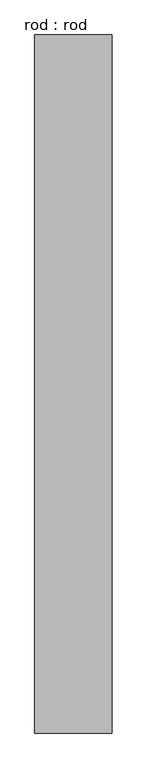
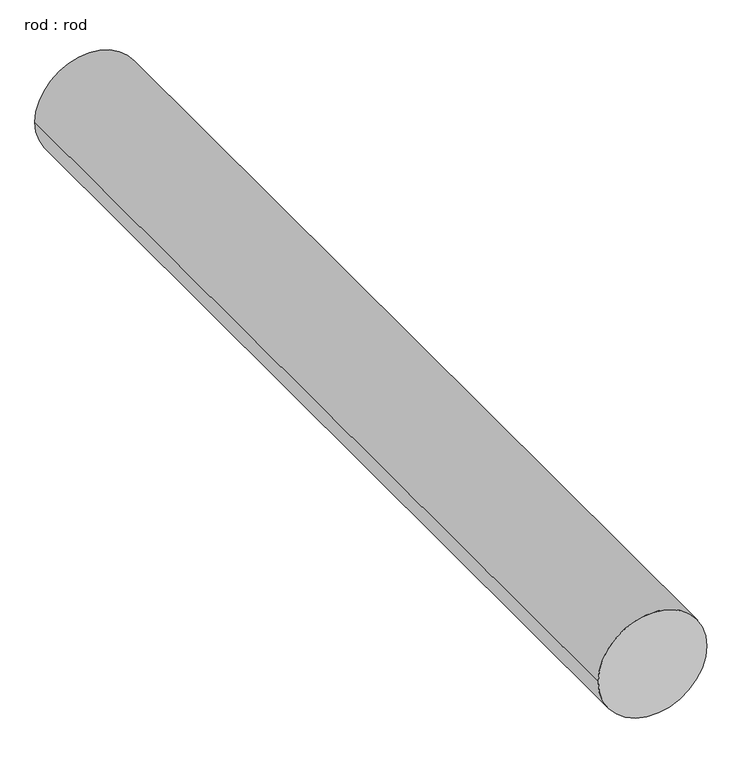
"""IFC4 building model written with IfcOpenShell, lengths in millimetres: proxy geometry, rod : rod."""

from ifc_helpers import new_model, si_unit, point, frame, frame_2d, origin, place, context, project, spatial, circle_curve, trimmed, segment, composite_curve, outline, extrude, source, transform, mapped, element, save


def rod_rod_469ef457(model_context):
    return source(origin(), model_context, "Body", "SweptSolid", [
        extrude(outline(composite_curve([segment(trimmed(circle_curve(frame_2d((0.0108462, 0.0)), 200.0), [point((0.0108462, 200.0))], [point((0.0108462, -200.0))], False, "CARTESIAN"), True, "CONTINUOUS"), segment(trimmed(circle_curve(frame_2d((0.0108462, 0.0)), 200.0), [point((0.0108462, -200.0))], [point((0.0108462, 200.0))], False, "CARTESIAN"), True, "CONTINUOUS")], self_intersect=False)), frame((0.0, 2292.7286153, 0.0), z_axis=(0.0, 1.0, 0.0), x_axis=(0.0, 0.0, 1.0)), (0.0, 0.0, 1.0), 3600.0),
    ])


if __name__ == "__main__":
    model = new_model("IFC4")
    model_context = context("Model", 3, world=origin())
    ifc_project = project(units=[si_unit("LENGTHUNIT", "METRE", prefix="MILLI")], contexts=[model_context])
    site = spatial("IfcSite", under=ifc_project)
    building = spatial("IfcBuilding", under=site)
    placement = place(None, origin())
    rod_rod_shape = rod_rod_469ef457(model_context)
    element("IfcBuildingElementProxy", 1, Name="rod : rod", ObjectType="rod : rod", at=placement, inside=building, context=model_context, shape_type="MappedRepresentation", body=[
        mapped(rod_rod_shape, transform((0.0, 0.0, 0.0), x_axis=(1.0, 0.0, 0.0), y_axis=(0.0, 1.0, 0.0), z_axis=(0.0, 0.0, 1.0))),
    ])
    save(model, "model.ifc")

# Revit data of these elements
# Type "rod : rod"
#   Default Elevation = 0
